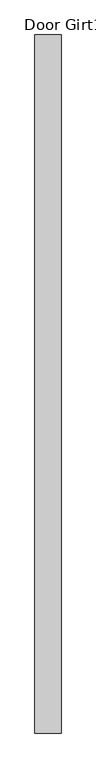
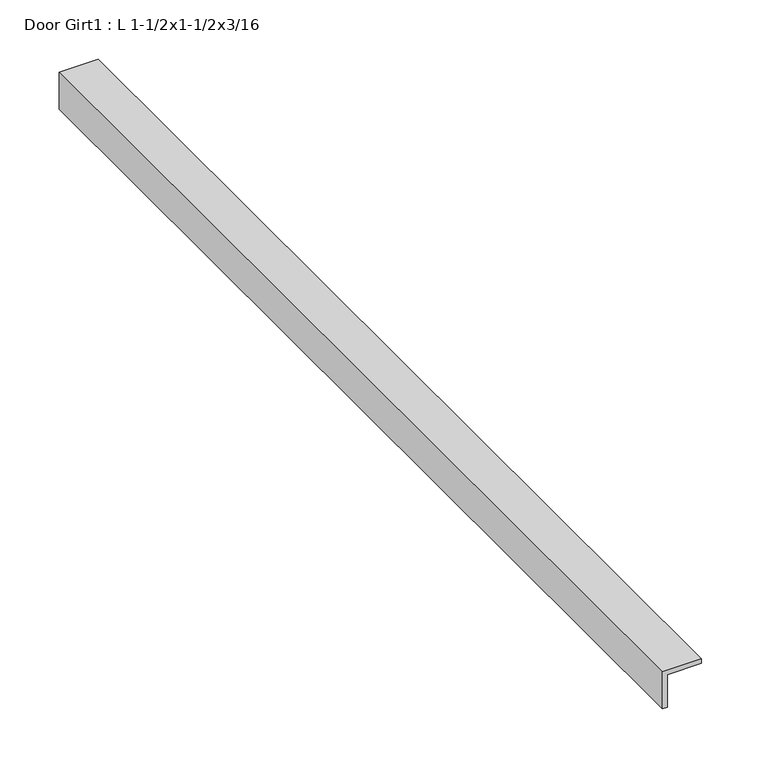
"""IFC4 building model written with IfcOpenShell, lengths in millimetres: proxy geometry, Door Girt1 : L 1-1/2x1-1/2x3/16."""

from ifc_helpers import new_model, si_unit, frame, origin, place, context, project, spatial, polyline, outline, extrude, source, transform, mapped, element, save


def door_girt1_l_1_1_2x1_1_2x3_16_7802d8c0(model_context):
    return source(origin(), model_context, "Body", "SweptSolid", [
        extrude(outline(polyline([(1625.6, 587403.9934739), (1625.6, 587365.8934739), (1587.5, 587365.8934739), (1587.5, 587370.6559739), (1620.8375, 587370.6559739), (1620.8375, 587403.9934739), (1625.6, 587403.9934739)])), frame((0.0, -535163.4663841, 0.0), z_axis=(0.0, 1.0, 0.0), x_axis=(0.0, 0.0, 1.0)), (0.0, 0.0, 1.0), 1017.5875),
    ])


if __name__ == "__main__":
    model = new_model("IFC4")
    model_context = context("Model", 3, world=origin())
    ifc_project = project(units=[si_unit("LENGTHUNIT", "METRE", prefix="MILLI")], contexts=[model_context])
    site = spatial("IfcSite", under=ifc_project)
    building = spatial("IfcBuilding", under=site)
    placement = place(None, origin())
    door_girt1_l_1_1_2x1_1_2x3_16_shape = door_girt1_l_1_1_2x1_1_2x3_16_7802d8c0(model_context)
    element("IfcBuildingElementProxy", 1, Name="Door Girt1 : L 1-1/2x1-1/2x3/16", ObjectType="Door Girt1 : L 1-1/2x1-1/2x3/16", at=placement, inside=building, context=model_context, shape_type="MappedRepresentation", body=[
        mapped(door_girt1_l_1_1_2x1_1_2x3_16_shape, transform((0.0, 0.0, 0.0), x_axis=(1.0, 0.0, 0.0), y_axis=(0.0, 1.0, 0.0), z_axis=(0.0, 0.0, 1.0))),
    ])
    save(model, "model.ifc")

# Revit data of these elements
# Element 1 (IfcBuildingElementProxy, "Door Girt1 : L 1-1/2x1-1/2x3/16")
#   Materials on its faces: "1-1/2\"X1-1/2\" GALV. STL L"
# Materials
#   "1-1/2\"X1-1/2\" GALV. STL L": class "Generic", colour RGB 211 211 207, transparency 0, Cost = 0
